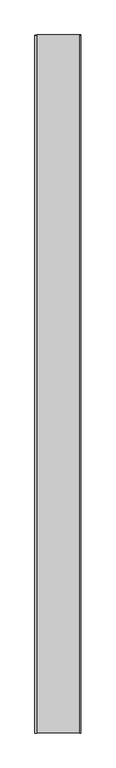
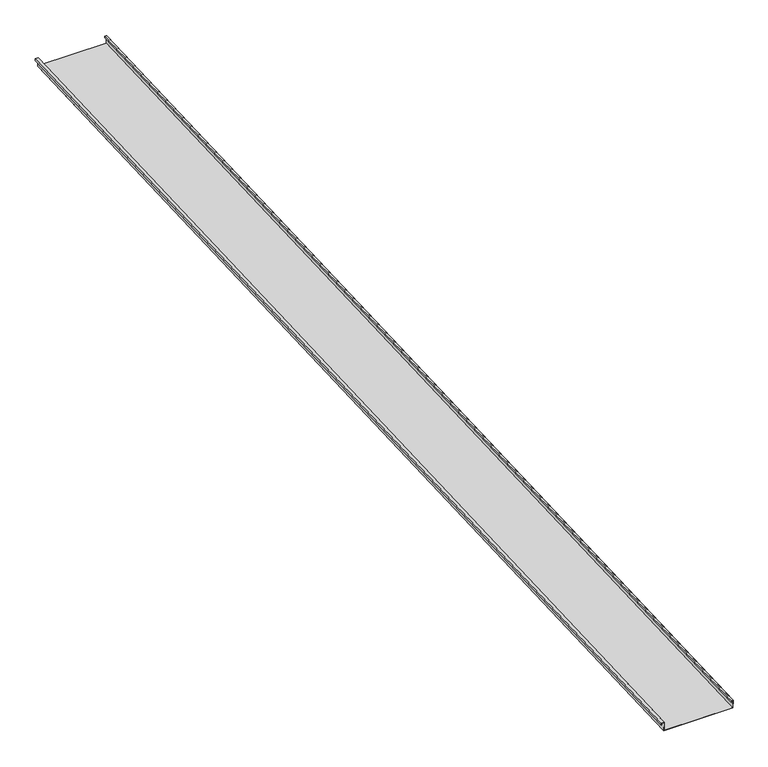
"""IFC4 building model written with IfcOpenShell, lengths in millimetres: proxy geometry, Generic Models 2:Generic Models 2:310765:Generic Models 2:310765 : Generic Models 2:Generic Models 2:310765:107 : Generic Models 2:Generic Models 2:310765:Generic Models 2:310765 : Generic Models 2:Generic Models 2:310765:300385."""

from ifc_helpers import new_model, si_unit, frame, origin, place, context, project, spatial, polyline, outline, extrude, source, transform, mapped, element, save


def generic_models_96411253(model_context):
    return source(origin(), model_context, "Body", "SweptSolid", [
        extrude(outline(polyline([(1.5875, 0.0), (1.5875, 50.8), (407.9875, 50.8), (407.9875, 1.5875), (396.875, 1.5875), (396.875, 11.1125), (398.4625, 11.1125), (398.4625, 3.175), (406.4, 3.175), (406.4, 49.2125), (3.175, 49.2125), (3.175, -1.5874999), (-14.2875, -1.5874999), (-14.2875, 9.525), (-12.7, 9.525), (-12.7, 0.0), (1.5875, 0.0)])), frame((610285.3929739, -581354.4345603, 3902.6697972), z_axis=(0.0, 0.9991330730923568, 0.041630544712067834), x_axis=(1.0, 0.0, 0.0)), (0.0, 0.0, 1.0), 6400.8),
    ])


if __name__ == "__main__":
    model = new_model("IFC4")
    model_context = context("Model", 3, world=origin())
    ifc_project = project(units=[si_unit("LENGTHUNIT", "METRE", prefix="MILLI")], contexts=[model_context])
    site = spatial("IfcSite", under=ifc_project)
    building = spatial("IfcBuilding", under=site)
    placement = place(None, origin())
    generic_models_shape = generic_models_96411253(model_context)
    element("IfcBuildingElementProxy", 1, Name="Generic Models 2:Generic Models 2:310765:Generic Models 2:310765 : Generic Models 2:Generic Models 2:310765:107 : Generic Models 2:Generic Models 2:310765:Generic Models 2:310765 : Generic Models 2:Generic Models 2:310765:300385", ObjectType="Generic Models 2:Generic Models 2:310765:Generic Models 2:310765 : Generic Models 2:Generic Models 2:310765:107 : Generic Models 2:Generic Models 2:310765:Generic Models 2:310765 : Generic Models 2:Generic Models 2:310765:300385", at=placement, inside=building, context=model_context, shape_type="MappedRepresentation", body=[
        mapped(generic_models_shape, transform((0.0, 0.0, 0.0), x_axis=(1.0, 0.0, 0.0), y_axis=(0.0, 1.0, 0.0), z_axis=(0.0, 0.0, 1.0))),
    ])
    save(model, "model.ifc")

# Revit data of these elements
# Type "Generic Models 2:Generic Models 2:310765:Generic Models 2:310765 : Generic Models 2:Generic Models 2:310765:107 : Generic Models 2:Generic Models 2:310765:Generic Models 2:310765 : Generic Models 2:Generic Models 2:310765:300385"
#   NameOverride = "Generic Models 2:Generic Models 2:310765:Generic Models 2:310765 : Generic Models 2:Generic Models 2:310765:300385"
#   ObjectTypeOverride = "Generic Models 2:310765 : Generic Models 2:Generic Models 2:310765"
#   Reference = "Generic Models 2"
#   Tag = "300385"
# Element 1 (IfcBuildingElementProxy, "Generic Models 2:Generic Models 2:310765:Generic Models 2:310765 : Generic Models 2:Generic Models 2:310765:107 : Generic Models 2:Generic Models 2:310765:Generic Models 2:310765 : Generic Models 2:Generic Models 2:310765:300385")
#   Materials on its faces: "THERMAL BROKEN ALUMINUM STOREFRONT FOR POLYCARBONATE"
# Materials
#   "THERMAL BROKEN ALUMINUM STOREFRONT FOR POLYCARBONATE": class "Unassigned", colour RGB 244 244 244, transparency 0, Keynote = "M07611300.01", Cost = 0
